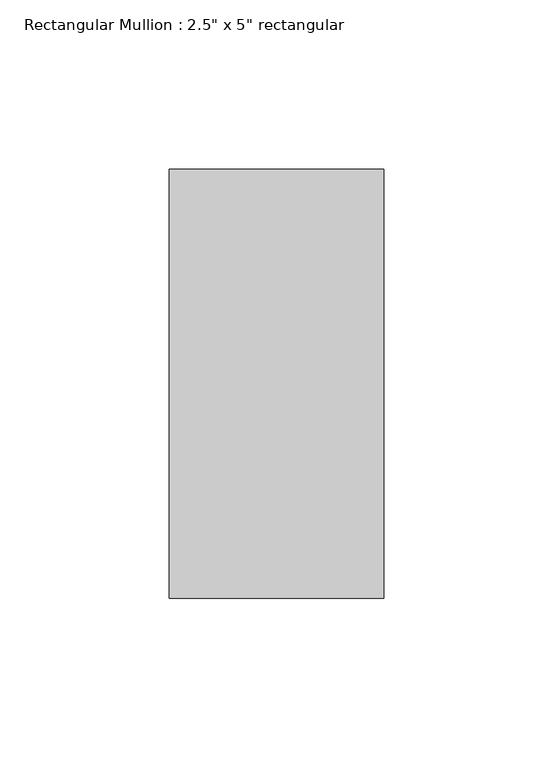
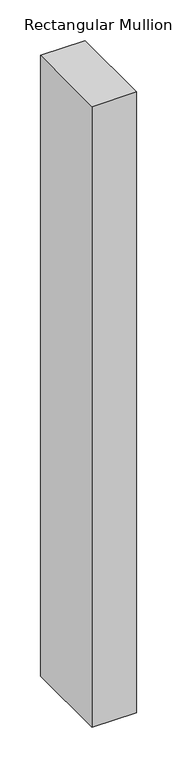
"""IFC4 building model written with IfcOpenShell, lengths in millimetres: member geometry."""

import ifcopenshell
import ifcopenshell.guid

model = None  # the IFC model being written
_history = None  # IfcOwnerHistory: only IFC2X3 demands one
_inside = {}  # id of a spatial element -> (the spatial element, [elements in it])
_under = {}  # id of a project, library or spatial element -> (it, [spatial elements below it])
_declared = {}  # id of a project -> (the project, [libraries it declares])
_typed = {}  # id of a type object -> (the type object, [elements of that type])
_made_of = {}  # id of a material, layer set ... -> (it, [elements and type objects made of it])


def new_model(schema):
    """Start an empty IFC model of exactly this schema.

    Asked for "IFC4X3", IfcOpenShell would pick the latest addendum, in which some entities
    have other attributes; the version numbers below select the first issue.
    IFC2X3 requires an IfcOwnerHistory on every rooted entity: one is made here for all.
    """
    global model, _history
    if schema == "IFC4X3":
        model = ifcopenshell.file(schema_version=(4, 3, 0, 0))
    else:
        model = ifcopenshell.file(schema=schema)
    _inside.clear()
    _under.clear()
    _declared.clear()
    _typed.clear()
    _made_of.clear()
    _history = None
    if model.schema == "IFC2X3":
        org = make("IfcOrganization", Name="unknown")
        user = make(
            "IfcPersonAndOrganization",
            ThePerson=make("IfcPerson", FamilyName="unknown"),
            TheOrganization=org,
        )
        app = make(
            "IfcApplication",
            ApplicationDeveloper=org,
            Version="unknown",
            ApplicationFullName="unknown",
            ApplicationIdentifier="unknown",
        )
        _history = make(
            "IfcOwnerHistory",
            OwningUser=user,
            OwningApplication=app,
            ChangeAction="ADDED",
            CreationDate=0,
        )
    return model


def make(cls, **values):
    """One entity of the class cls with the attributes given. An attribute that is None is left unset."""
    return model.create_entity(
        cls, **{name: value for name, value in values.items() if value is not None}
    )


def rooted(cls, **values):
    """An entity with a GlobalId (a new one), such as an element, a storey or a relation."""
    return make(cls, GlobalId=ifcopenshell.guid.new(), OwnerHistory=_history, **values)


def si_unit(unit_type, name, prefix=None):
    """IfcSIUnit, for example si_unit("LENGTHUNIT", "METRE", prefix="MILLI")."""
    return make("IfcSIUnit", UnitType=unit_type, Prefix=prefix, Name=name)


def assignment(units):
    """IfcUnitAssignment: the units of a project."""
    return None if units is None else make("IfcUnitAssignment", Units=units)


def point(xyz):
    """IfcCartesianPoint."""
    return None if xyz is None else make("IfcCartesianPoint", Coordinates=xyz)


def direction(xyz):
    """IfcDirection."""
    return None if xyz is None else make("IfcDirection", DirectionRatios=xyz)


def frame(location, z_axis=None, x_axis=None):
    """IfcAxis2Placement3D, a coordinate frame: its origin and axes. An axis left out is left unset."""
    return make(
        "IfcAxis2Placement3D",
        Location=point(location),
        Axis=direction(z_axis),
        RefDirection=direction(x_axis),
    )


def origin():
    """The frame at (0, 0, 0) with its axes left unset."""
    return frame((0.0, 0.0, 0.0))


def place(relative_to, where):
    """IfcLocalPlacement: puts the frame where relative to a parent placement (None: the world)."""
    return make(
        "IfcLocalPlacement", PlacementRelTo=relative_to, RelativePlacement=where
    )


def context(
    kind, dimensions, precision=None, world=None, true_north=None, identifier=None
):
    """IfcGeometricRepresentationContext, for example the 3D "Model" context."""
    return make(
        "IfcGeometricRepresentationContext",
        ContextIdentifier=identifier,
        ContextType=kind,
        CoordinateSpaceDimension=dimensions,
        Precision=precision,
        WorldCoordinateSystem=world,
        TrueNorth=true_north,
    )


def project(units=None, contexts=None):
    """IfcProject with its units and contexts."""
    return rooted(
        "IfcProject",
        Name="project",
        RepresentationContexts=contexts,
        UnitsInContext=assignment(units),
    )


def spatial(cls, under=None, at=None, **own):
    """A site, building, storey or space (cls), placed at a placement, below another one or the project."""
    s = rooted(cls, ObjectPlacement=at, **own)
    if under is not None:
        _under.setdefault(under.id(), (under, []))[1].append(s)
    return s


def polyline(points):
    """IfcPolyline through the points."""
    return make("IfcPolyline", Points=[point(p) for p in points])


def outline(outer, holes=None, kind="AREA"):
    """IfcArbitraryClosedProfileDef: a profile drawn as a closed curve; with holes, ...WithVoids."""
    if holes is None:
        return make("IfcArbitraryClosedProfileDef", ProfileType=kind, OuterCurve=outer)
    return make(
        "IfcArbitraryProfileDefWithVoids",
        ProfileType=kind,
        OuterCurve=outer,
        InnerCurves=holes,
    )


def extrude(swept, where, along, depth):
    """IfcExtrudedAreaSolid: the profile swept, set in the frame where, extruded along a direction by depth."""
    return make(
        "IfcExtrudedAreaSolid",
        SweptArea=swept,
        Position=where,
        ExtrudedDirection=direction(along),
        Depth=depth,
    )


def shape(context_of_items, identifier, shape_type, items):
    """IfcShapeRepresentation: the items that make up one representation, for example the "Body"."""
    return make(
        "IfcShapeRepresentation",
        ContextOfItems=context_of_items,
        RepresentationIdentifier=identifier,
        RepresentationType=shape_type,
        Items=items,
    )


def source(mapping_origin, context_of_items, identifier, shape_type, items):
    """IfcRepresentationMap: a shape defined once, which mapped items show again and again."""
    return make(
        "IfcRepresentationMap",
        MappingOrigin=mapping_origin,
        MappedRepresentation=shape(context_of_items, identifier, shape_type, items),
    )


def transform(
    local_origin,
    x_axis=None,
    y_axis=None,
    z_axis=None,
    scale=None,
    scale2=None,
    scale3=None,
    uniform=True,
):
    """IfcCartesianTransformationOperator3D, or its non-uniform kind. x_axis, y_axis, z_axis: its Axis1, 2, 3."""
    if uniform:
        return make(
            "IfcCartesianTransformationOperator3D",
            Axis1=direction(x_axis),
            Axis2=direction(y_axis),
            LocalOrigin=point(local_origin),
            Scale=scale,
            Axis3=direction(z_axis),
        )
    return make(
        "IfcCartesianTransformationOperator3DnonUniform",
        Axis1=direction(x_axis),
        Axis2=direction(y_axis),
        LocalOrigin=point(local_origin),
        Scale=scale,
        Axis3=direction(z_axis),
        Scale2=scale2,
        Scale3=scale3,
    )


def mapped(mapping_source, mapping_target):
    """IfcMappedItem: shows the shape of a source again, moved by a transform."""
    return make(
        "IfcMappedItem", MappingSource=mapping_source, MappingTarget=mapping_target
    )


def made_of(thing, what):
    """Note that an element or type object is made of a material, layer set ...; save() writes the relation."""
    if what is not None:
        _made_of.setdefault(what.id(), (what, []))[1].append(thing)
    return thing


def element(
    cls,
    number,
    at=None,
    inside=None,
    cuts=None,
    type_object=None,
    material=None,
    context=None,
    identifier="Body",
    shape_type=None,
    held_by="IfcProductDefinitionShape",
    body=None,
    shapes=None,
    **own,
):
    """One element of the class cls, such as IfcWall. Its Tag is "e" and its number.

    at: its placement. inside: the storey or other place that contains it. cuts: it is an
    opening in that element (IfcRelVoidsElement). A single representation is given by context,
    identifier, shape_type and body (its items); several are given by shapes. held_by: the class
    of the entity that holds the representations. save() writes the other relations.
    """
    e = rooted(cls, Tag="e%d" % number, ObjectPlacement=at, **own)
    if body is not None:
        shapes = [shape(context, identifier, shape_type, body)]
    if shapes is not None:
        e.Representation = make(held_by, Representations=shapes)
    if inside is not None:
        _inside.setdefault(inside.id(), (inside, []))[1].append(e)
    if cuts is not None:
        rooted(
            "IfcRelVoidsElement", RelatingBuildingElement=cuts, RelatedOpeningElement=e
        )
    if type_object is not None:
        _typed.setdefault(type_object.id(), (type_object, []))[1].append(e)
    return made_of(e, material)


def aggregate(whole, parts):
    """IfcRelAggregates: a whole, such as a stair, and the parts it consists of."""
    return rooted("IfcRelAggregates", RelatingObject=whole, RelatedObjects=parts)


def save(model, path):
    """Write the relations noted so far, then the file.

    IfcRelAggregates (storeys below a building ...), IfcRelContainedInSpatialStructure (elements
    in a storey), IfcRelDefinesByType, IfcRelAssociatesMaterial and IfcRelDeclares: one each for
    every whole, place, type object, material and project.
    """
    for whole, parts in _under.values():
        aggregate(whole, parts)
    for where, things in _inside.values():
        rooted(
            "IfcRelContainedInSpatialStructure",
            RelatedElements=things,
            RelatingStructure=where,
        )
    for kind, things in _typed.values():
        rooted("IfcRelDefinesByType", RelatedObjects=things, RelatingType=kind)
    for what, things in _made_of.values():
        rooted("IfcRelAssociatesMaterial", RelatedObjects=things, RelatingMaterial=what)
    for by, libraries in _declared.values():
        rooted("IfcRelDeclares", RelatingContext=by, RelatedDefinitions=libraries)
    model.write(path)


def member_03f32644(model_context):
    return source(origin(), model_context, "Body", "SweptSolid", [
        extrude(outline(polyline([(0.0, 63.5), (0.0, -63.5), (-63.5, -63.5), (-63.5, 63.5), (0.0, 63.5)])), frame((0.0, 0.0, -933.4500001), z_axis=(0.0, 0.0, 1.0), x_axis=(1.0, 0.0, 0.0)), (0.0, 0.0, 1.0), 933.4500001),
    ])


if __name__ == "__main__":
    model = new_model("IFC4")
    model_context = context("Model", 3, world=origin())
    ifc_project = project(units=[si_unit("LENGTHUNIT", "METRE", prefix="MILLI")], contexts=[model_context])
    site = spatial("IfcSite", under=ifc_project)
    building = spatial("IfcBuilding", under=site)
    placement = place(None, origin())
    member_shape = member_03f32644(model_context)
    element("IfcMember", 1, ObjectType="Rectangular Mullion : 2.5\" x 5\" rectangular", at=placement, inside=building, context=model_context, shape_type="MappedRepresentation", body=[
        mapped(member_shape, transform((0.0, 0.0, 0.0), x_axis=(1.0, 0.0, 0.0), y_axis=(0.0, 1.0, 0.0), z_axis=(0.0, 0.0, 1.0))),
    ])
    save(model, "model.ifc")

# Revit data of these elements
# Type "Rectangular Mullion : 2.5\" x 5\" rectangular"
#   built-in parameter 1007304 = 0.416667 (stored number, unit not read)
#   built-in parameter 1007301 = 0.104167 (stored number, unit not read)
#   built-in parameter 1007300 = 0.104167 (stored number, unit not read)
# Element 1 (IfcMember, "Rectangular Mullion : 2.5\" x 5\" rectangular")
#   Materials on its faces: "Aluminum"
# Materials
#   "Aluminum": class "Metal", colour RGB 247 247 247, transparency 0, Description = "Aluminum 6061", Cost = 0
